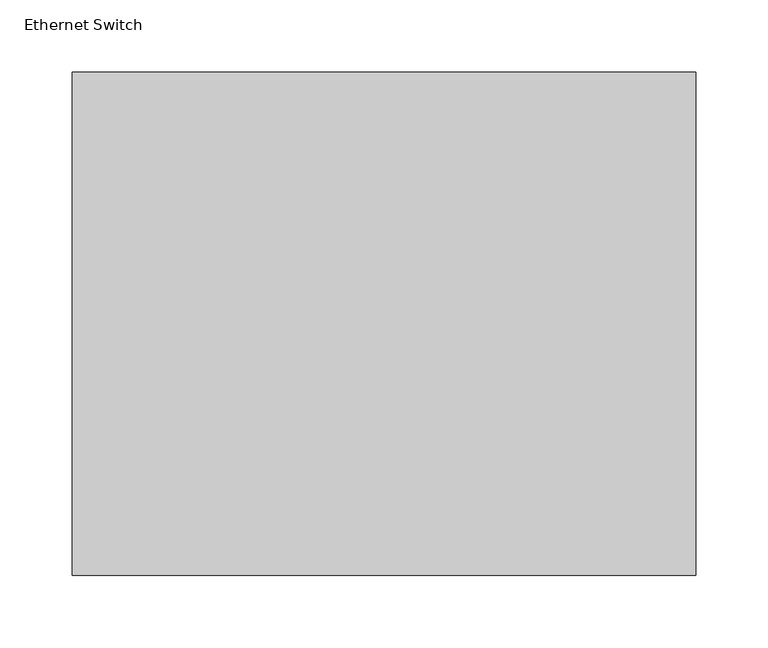
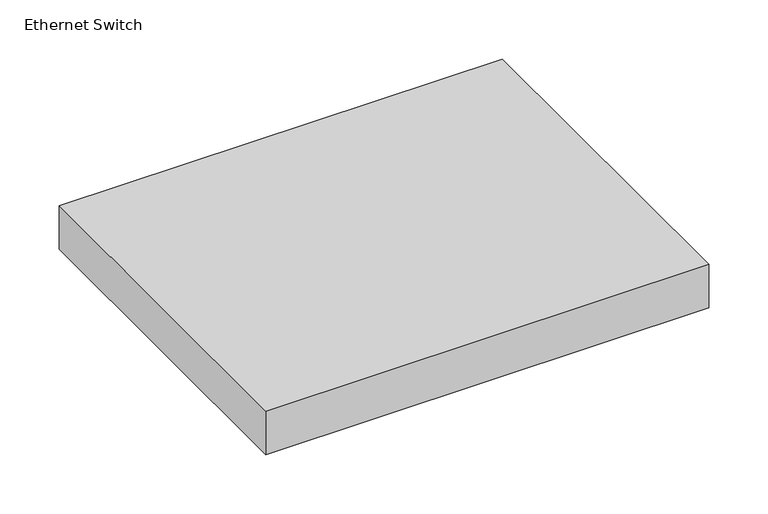
"""IFC4 building model written with IfcOpenShell, lengths in millimetres: proxy geometry, Ethernet Switch : NETGEAR 16 Port Gigabit Ethernet Plus Network Switch (GS116E)."""

from ifc_helpers import new_model, si_unit, origin, origin_with_axes, place, context, project, spatial, polyline, outline, extrude, source, transform, mapped, element, save


def ethernet_switch_5c8040eb(model_context):
    return source(origin(), model_context, "Body", "SweptSolid", [
        extrude(outline(polyline([(216.05, 174.5), (216.05, -174.5), (-216.05, -174.5), (-216.05, 174.5), (216.05, 174.5)])), origin_with_axes(), (0.0, 0.0, 1.0), 44.9),
    ])


if __name__ == "__main__":
    model = new_model("IFC4")
    model_context = context("Model", 3, world=origin())
    ifc_project = project(units=[si_unit("LENGTHUNIT", "METRE", prefix="MILLI")], contexts=[model_context])
    site = spatial("IfcSite", under=ifc_project)
    building = spatial("IfcBuilding", under=site)
    placement = place(None, origin())
    ethernet_switch_shape = ethernet_switch_5c8040eb(model_context)
    element("IfcBuildingElementProxy", 1, Name="Ethernet Switch : NETGEAR 16 Port Gigabit Ethernet Plus Network Switch (GS116E)", ObjectType="Ethernet Switch : NETGEAR 16 Port Gigabit Ethernet Plus Network Switch (GS116E)", at=placement, inside=building, context=model_context, shape_type="MappedRepresentation", body=[
        mapped(ethernet_switch_shape, transform((0.0, 0.0, 0.0), x_axis=(1.0, 0.0, 0.0), y_axis=(0.0, 1.0, 0.0), z_axis=(0.0, 0.0, 1.0))),
    ])
    save(model, "model.ifc")

# Revit data of these elements
# Project information
#   Document_Suitability_Code = "A1"
#   Document_Suitability_Description = "Construction"
#   Project Issue Date = "Oct 2020"
#   Project Status = "Project Status"
#   Client Name = "Your Name Here"
#   Project Address = "Enter address here"
#   Project Name = "Revit MEP 01"
#   Project Number = "RMEP01"
# Type "Ethernet Switch : NETGEAR 16 Port Gigabit Ethernet Plus Network Switch (GS116E)"
#   Width = 432.1 mm
#   Height = 44.9 mm
#   Depth = 349 mm
#   built-in parameter 1140087 [instance default] = 1
#   Default Elevation = 0
